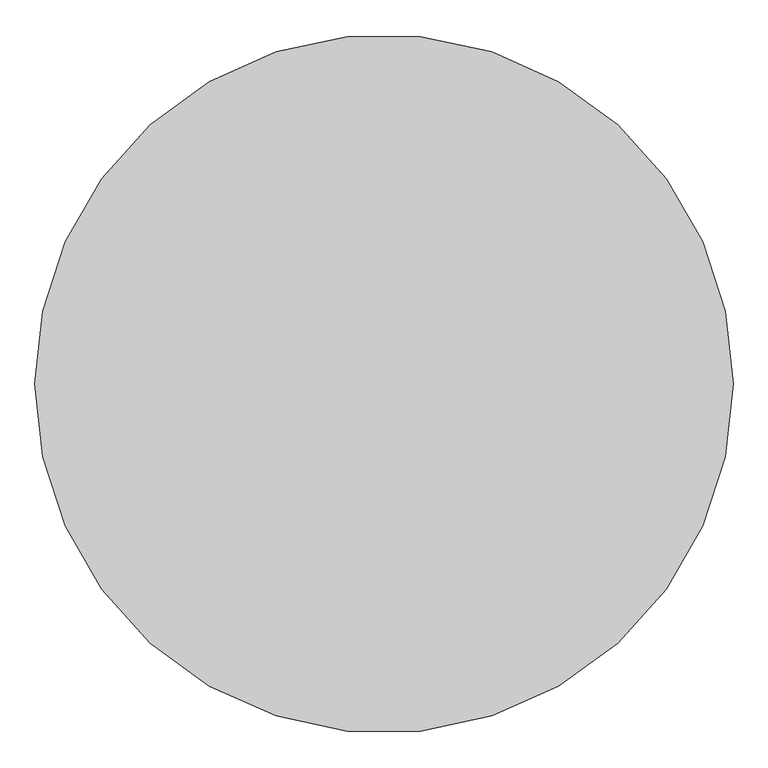
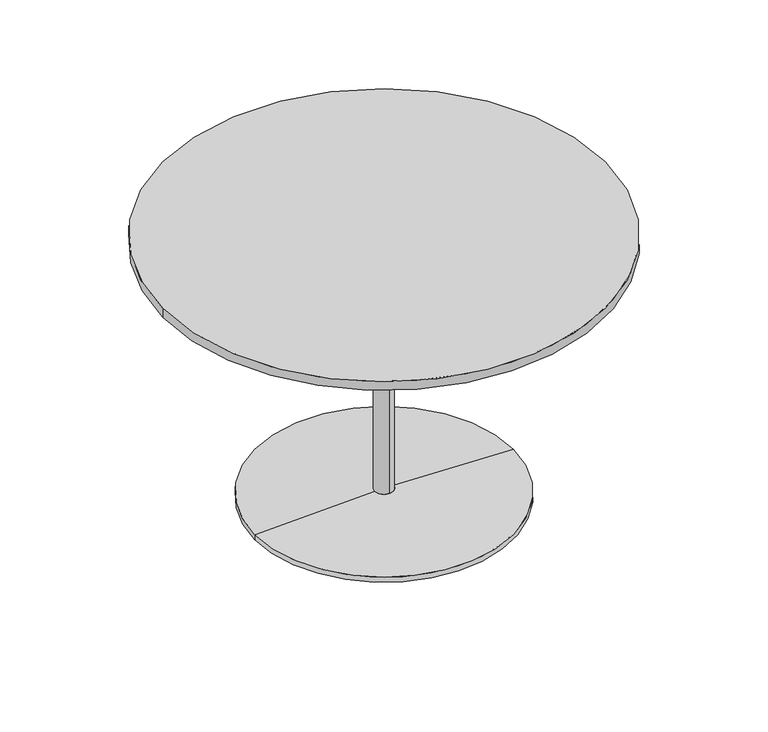
"""IFC4 building model written with IfcOpenShell, lengths in millimetres: furniture geometry, Table, Round-NON-COLLECTUS : -."""

from ifc_helpers import new_model, si_unit, point, frame, frame_2d, origin, origin_2d, place, context, project, spatial, polyline, circle_curve, trimmed, segment, composite_curve, outline, extrude, source, transform, mapped, element, save
from ifc_brep_helpers import plane_surface, cylinder_surface, revolved_surface, advanced_brep


def furniture_29bad768(model_context):
    return source(origin(), model_context, "Body", "SolidModel", [
        extrude(outline(composite_curve([segment(trimmed(circle_curve(frame_2d((-0.4435274, 0.0)), 25.4), [point((-0.4435274, 25.4))], [point((-0.4435274, -25.4))], False, "CARTESIAN"), True, "CONTINUOUS"), segment(trimmed(circle_curve(frame_2d((-0.4435274, 0.0)), 25.4), [point((-0.4435274, -25.4))], [point((-0.4435274, 25.4))], False, "CARTESIAN"), True, "CONTINUOUS")], self_intersect=False)), frame((0.0, 0.0, 25.4), z_axis=(0.0, 0.0, 1.0), x_axis=(1.0, 0.0, 0.0)), (0.0, 0.0, 1.0), 711.2),
        advanced_brep(
        [(0.0, 0.0, 0.0), (-355.6, 0.0, 0.0), (355.6, 0.0, 0.0), (25.4, 0.0, 25.4), (-25.4, 0.0, 25.4), (0.0, 0.0, 25.4), (355.6, 0.0, 14.5873178), (-355.6, 0.0, 14.5873178)],
        [
            (0, 1),
            (1, 2, circle_curve(frame((0.0, 0.0, 0.0), z_axis=(0.0, 0.0, -1.0), x_axis=(-1.0, 0.0, 0.0)), 355.6)),
            (2, 0),
            (2, 1, circle_curve(frame((0.0, 0.0, 0.0), z_axis=(0.0, 0.0, -1.0), x_axis=(-1.0, 0.0, 0.0)), 355.6)),
            (3, 4, circle_curve(frame((0.0, 0.0, 25.4), z_axis=(0.0, 0.0, 1.0), x_axis=(-1.0, 0.0, 0.0)), 25.4)),
            (4, 5),
            (5, 3),
            (4, 3, circle_curve(frame((0.0, 0.0, 25.4), z_axis=(0.0, 0.0, 1.0), x_axis=(-1.0, 0.0, 0.0)), 25.4)),
            (6, 7, circle_curve(frame((0.0, 0.0, 14.5873178), z_axis=(0.0, 0.0, 1.0), x_axis=(-1.0, 0.0, 0.0)), 355.6)),
            (7, 4),
            (3, 6),
            (7, 6, circle_curve(frame((0.0, 0.0, 14.5873178), z_axis=(0.0, 0.0, 1.0), x_axis=(-1.0, 0.0, 0.0)), 355.6)),
            (1, 7),
            (6, 2),
        ],
        [
            plane_surface(frame((0.0, 0.0, 0.0), z_axis=(0.0, 0.0, -1.0), x_axis=(-1.0, 0.0, 0.0))),
            plane_surface(frame((0.0, 0.0, 25.4), z_axis=(0.0, 0.0, 1.0), x_axis=(-1.0, 0.0, 0.0))),
            revolved_surface(polyline([(-25.4, 0.0, 25.4), (-355.6, 0.0, 14.5873178)]), (0.0, 0.0, 57.15), (0.0, 0.0, -1.0)),
            cylinder_surface(frame((0.0, 0.0, 57.15), z_axis=(0.0, 0.0, -1.0), x_axis=(-1.0, 0.0, 0.0)), 355.6),
        ],
        [
            (0, [[1, 2, 3]]),
            (0, [[-3, 4, -1]]),
            (1, [[5, 6, 7]]),
            (1, [[8, -7, -6]]),
            (2, [[9, 10, -5, 11]]),
            (2, [[12, -11, -8, -10]]),
            (3, [[-2, 13, -9, 14]]),
            (3, [[-4, -14, -12, -13]]),
        ],
    ),
        extrude(outline(composite_curve([segment(trimmed(circle_curve(origin_2d(), 609.6), [point((609.6, 0.0))], [point((-609.6, 0.0))], False, "CARTESIAN"), True, "CONTINUOUS"), segment(trimmed(circle_curve(origin_2d(), 609.6), [point((-609.6, 0.0))], [point((609.6, 0.0))], False, "CARTESIAN"), True, "CONTINUOUS")], self_intersect=False)), frame((0.0, 0.0, 736.6), z_axis=(0.0, 0.0, 1.0), x_axis=(1.0, 0.0, 0.0)), (0.0, 0.0, 1.0), 25.4),
    ])


if __name__ == "__main__":
    model = new_model("IFC4")
    model_context = context("Model", 3, world=origin())
    ifc_project = project(units=[si_unit("LENGTHUNIT", "METRE", prefix="MILLI")], contexts=[model_context])
    site = spatial("IfcSite", under=ifc_project)
    building = spatial("IfcBuilding", under=site)
    placement = place(None, origin())
    furniture_shape = furniture_29bad768(model_context)
    element("IfcFurniture", 1, ObjectType="Table, Round-NON-COLLECTUS : -", at=placement, inside=building, context=model_context, shape_type="MappedRepresentation", body=[
        mapped(furniture_shape, transform((0.0, 0.0, 0.0), x_axis=(1.0, 0.0, 0.0), y_axis=(0.0, 1.0, 0.0), z_axis=(0.0, 0.0, 1.0))),
    ])
    save(model, "model.ifc")

# Revit data of these elements
# Type "Table, Round-NON-COLLECTUS : -"
#   External ID [instance default] = ""
#   Width = 1219.2 mm
#   Radius = 609.6 mm
#   Height = 762 mm
#   Depth = 1219.2 mm
#   OBO White = White
#   Default Elevation = 0
# Element 1 (IfcFurniture, "Table, Round-NON-COLLECTUS : -")
#   Materials on its faces: "White"
# Materials
#   "White": class "Generic", colour RGB 255 255 255, transparency 0, Cost = 0
